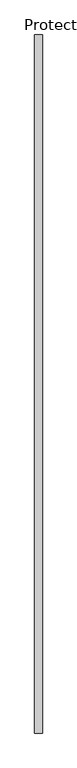
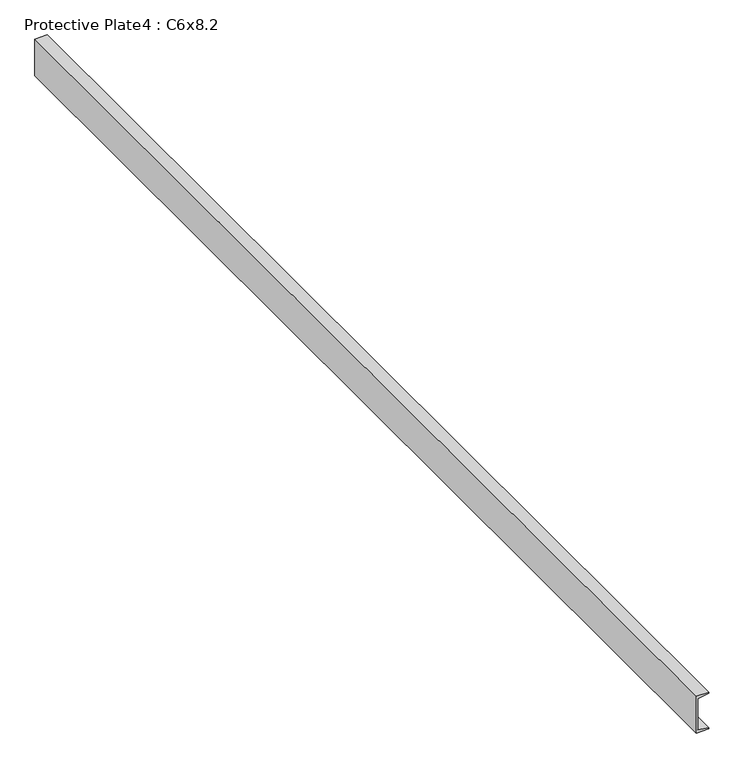
"""IFC4 building model written with IfcOpenShell, lengths in millimetres: proxy geometry, Protective Plate4 : C6x8.2."""

from ifc_helpers import new_model, si_unit, frame, origin, place, context, project, spatial, polyline, outline, extrude, source, transform, mapped, element, save


def protective_plate4_c6x8_2_0a73d697(model_context):
    return source(origin(), model_context, "Body", "SweptSolid", [
        extrude(outline(polyline([(914.4, 590217.0434739), (914.4, 590168.2754739), (762.0, 590168.2754739), (762.0, 590217.0434739), (767.08, 590217.0434739), (774.7868721, 590173.3356302), (901.6131279, 590173.3356302), (909.32, 590217.0434739), (914.4, 590217.0434739)])), frame((0.0, -536297.9573841, 0.0), z_axis=(0.0, 1.0, 0.0), x_axis=(0.0, 0.0, 1.0)), (0.0, 0.0, 1.0), 4473.448),
    ])


if __name__ == "__main__":
    model = new_model("IFC4")
    model_context = context("Model", 3, world=origin())
    ifc_project = project(units=[si_unit("LENGTHUNIT", "METRE", prefix="MILLI")], contexts=[model_context])
    site = spatial("IfcSite", under=ifc_project)
    building = spatial("IfcBuilding", under=site)
    placement = place(None, origin())
    protective_plate4_c6x8_2_shape = protective_plate4_c6x8_2_0a73d697(model_context)
    element("IfcBuildingElementProxy", 1, Name="Protective Plate4 : C6x8.2", ObjectType="Protective Plate4 : C6x8.2", at=placement, inside=building, context=model_context, shape_type="MappedRepresentation", body=[
        mapped(protective_plate4_c6x8_2_shape, transform((0.0, 0.0, 0.0), x_axis=(1.0, 0.0, 0.0), y_axis=(0.0, 1.0, 0.0), z_axis=(0.0, 0.0, 1.0))),
    ])
    save(model, "model.ifc")

# Revit data of these elements
# Element 1 (IfcBuildingElementProxy, "Protective Plate4 : C6x8.2")
#   Materials on its faces: "C6x8.2 GALV CHANNEL"
# Materials
#   "C6x8.2 GALV CHANNEL": class "Generic", colour RGB 211 211 207, transparency 0, Cost = 0
